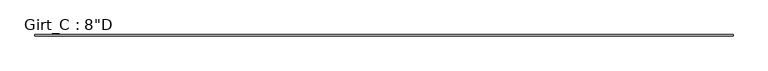
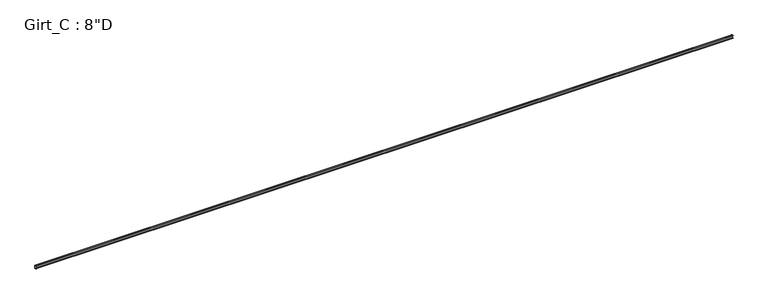
"""IFC4 building model written with IfcOpenShell, lengths in millimetres: beam geometry."""

from ifc_helpers import new_model, si_unit, point, frame, frame_2d, origin, place, context, project, spatial, polyline, circle_curve, trimmed, segment, composite_curve, outline, extrude, source, transform, mapped, element, save


def beam_4f0685ea(model_context):
    return source(origin(), model_context, "Body", "SweptSolid", [
        extrude(outline(composite_curve([segment(polyline([(-87.5109375, 101.6), (-3.3734375, 101.6)]), True, "CONTINUOUS"), segment(trimmed(circle_curve(frame_2d((-3.3734375, 96.8375)), 4.7625), [point((-3.3734375, 101.6))], [point((1.3890625, 96.8375))], False, "CARTESIAN"), True, "CONTINUOUS"), segment(polyline([(1.3890625, 96.8375), (1.3890625, -96.8375)]), True, "CONTINUOUS"), segment(trimmed(circle_curve(frame_2d((-3.3734375, -96.8375)), 4.7625), [point((1.3890625, -96.8375))], [point((-3.3734375, -101.6))], False, "CARTESIAN"), True, "CONTINUOUS"), segment(polyline([(-3.3734375, -101.6), (-87.5109375, -101.6), (-99.7792647, -86.979177), (-97.6510975, -85.1934327), (-86.2154765, -98.821875), (-3.2694106, -98.821875)]), True, "CONTINUOUS"), segment(trimmed(circle_curve(frame_2d((-3.3748024, -96.8389339)), 1.9857399), [point((-3.2694106, -98.821875))], [point((-1.3890625, -96.8389339))], True, "CARTESIAN"), True, "CONTINUOUS"), segment(polyline([(-1.3890625, -96.8389339), (-1.3890625, 96.8381931)]), True, "CONTINUOUS"), segment(trimmed(circle_curve(frame_2d((-3.3741066, 96.8381931)), 1.9850441), [point((-1.3890625, 96.8381931))], [point((-3.3005807, 98.821875))], True, "CARTESIAN"), True, "CONTINUOUS"), segment(polyline([(-3.3005807, 98.821875), (-86.2154765, 98.821875), (-97.6278742, 85.221109), (-99.7560415, 87.0068534), (-87.5109375, 101.6)]), True, "CONTINUOUS")], self_intersect=False)), frame((-23923.625, 0.0, 0.0), z_axis=(1.0, 0.0, 0.0), x_axis=(0.0, 1.0, 0.0)), (0.0, 0.0, 1.0), 47847.25),
    ])


if __name__ == "__main__":
    model = new_model("IFC4")
    model_context = context("Model", 3, world=origin())
    ifc_project = project(units=[si_unit("LENGTHUNIT", "METRE", prefix="MILLI")], contexts=[model_context])
    site = spatial("IfcSite", under=ifc_project)
    building = spatial("IfcBuilding", under=site)
    placement = place(None, origin())
    beam_shape = beam_4f0685ea(model_context)
    element("IfcBeam", 1, ObjectType="Girt_C : 8\"D", at=placement, inside=building, context=model_context, shape_type="MappedRepresentation", body=[
        mapped(beam_shape, transform((0.0, 0.0, 0.0), x_axis=(1.0, 0.0, 0.0), y_axis=(0.0, 1.0, 0.0), z_axis=(0.0, 0.0, 1.0))),
    ])
    save(model, "model.ifc")

# Revit data of these elements
# Type "Girt_C : 8\"D"
#   half leg = 0' - 1 3/4"
#   Web_Thickness = 0' - 0 7/64"
#   Length [instance default] = 10' - 0"
#   Leg_1 = 0' - 3 1/2"
#   Height = 0' - 8"
#   Structural Material [instance default] = none
# Element 1 (IfcBeam, "Girt_C : 8\"D")
#   Structural Material = CEE' SECTION (8.0x3.5C - SEE STRUCT. DWGS)
#   Materials on its faces: "CEE' SECTION (8.0x3.5C - SEE STRUCT. DWGS)"
# Materials
#   "CEE' SECTION (8.0x3.5C - SEE STRUCT. DWGS)": class "Metal", colour RGB 137 146 153, transparency 0, Description = "Steel, mill finish", Cost = 0
